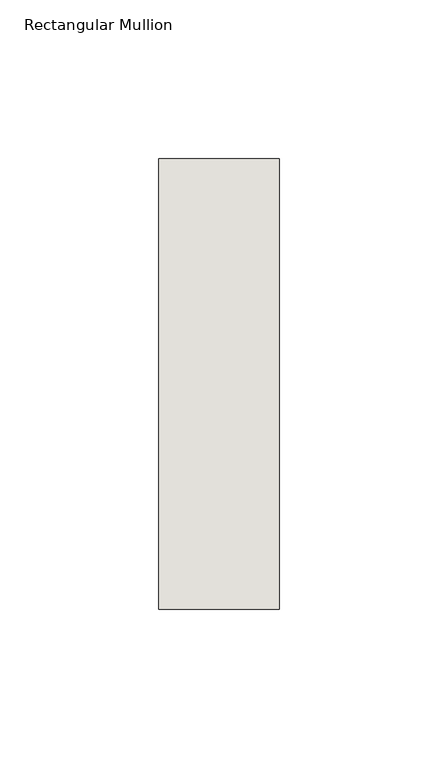
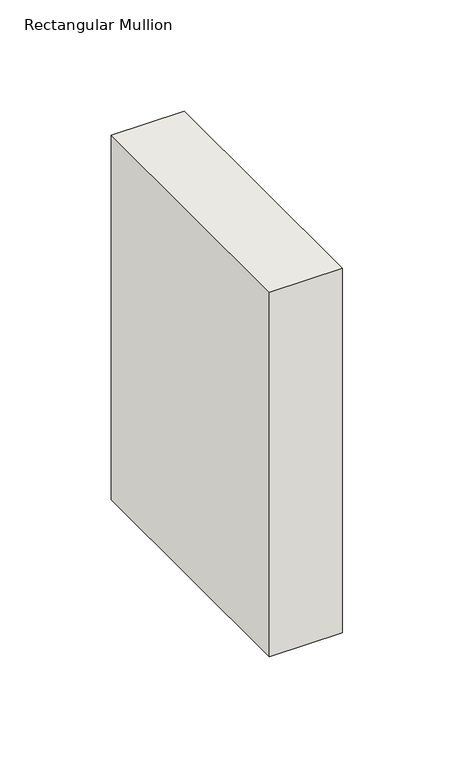
"""IFC4 building model written with IfcOpenShell, lengths in millimetres: wall geometry, Rectangular Mullion : NLRS_21_CWM_hsb-regel 38x142_gen_rsf."""

from ifc_helpers import new_model, si_unit, frame, origin, place, context, project, spatial, polyline, outline, extrude, source, transform, mapped, element, save


def rectangular_mullion_cea15bcf(model_context):
    return source(origin(), model_context, "Body", "SweptSolid", [
        extrude(outline(polyline([(-38.0, -71.0), (-38.0, 71.0), (0.0, 71.0), (0.0, -71.0), (-38.0, -71.0)])), frame((0.0, 0.0, -199.9999997), z_axis=(0.0, 0.0, 1.0), x_axis=(1.0, 0.0, 0.0)), (0.0, 0.0, 1.0), 199.9999997),
    ])


if __name__ == "__main__":
    model = new_model("IFC4")
    model_context = context("Model", 3, world=origin())
    ifc_project = project(units=[si_unit("LENGTHUNIT", "METRE", prefix="MILLI")], contexts=[model_context])
    site = spatial("IfcSite", under=ifc_project)
    building = spatial("IfcBuilding", under=site)
    placement = place(None, origin())
    rectangular_mullion_shape = rectangular_mullion_cea15bcf(model_context)
    element("IfcWall", 1, ObjectType="Rectangular Mullion : NLRS_21_CWM_hsb-regel 38x142_gen_rsf", at=placement, inside=building, context=model_context, shape_type="MappedRepresentation", body=[
        mapped(rectangular_mullion_shape, transform((0.0, 0.0, 0.0), x_axis=(1.0, 0.0, 0.0), y_axis=(0.0, 1.0, 0.0), z_axis=(0.0, 0.0, 1.0))),
    ])
    save(model, "model.ifc")

# Revit data of these elements
# Type "Rectangular Mullion : NLRS_21_CWM_hsb-regel 38x142_gen_rsf"
#   Type IfcGUID = "07M7mRoiH1CR8m_RSKIwpF"
#   Assembly Code = "21.10"
#   IfcExportAs = "IfcWall"
#   built-in parameter 1007322 = 0.465879 (stored number, unit not read)
#   built-in parameter 1007321 = 0.062336 (stored number, unit not read)
#   built-in parameter 1007320 = 0.062336 (stored number, unit not read)
# Element 1 (IfcWall, "Rectangular Mullion : NLRS_21_CWM_hsb-regel 38x142_gen_rsf")
#   Materials on its faces: "NLRS_i2_hout naaldhout vuren_gen_rsf"
# Materials
#   "NLRS_i2_hout naaldhout vuren_gen_rsf": class "I - Hout", colour RGB 234 199 147, transparency 0, Keynote = "i2", Manufacturer = "Revit Standards Foundation", URL = "www.revitstandards.org", Description = "hout vuren", Cost = 0
